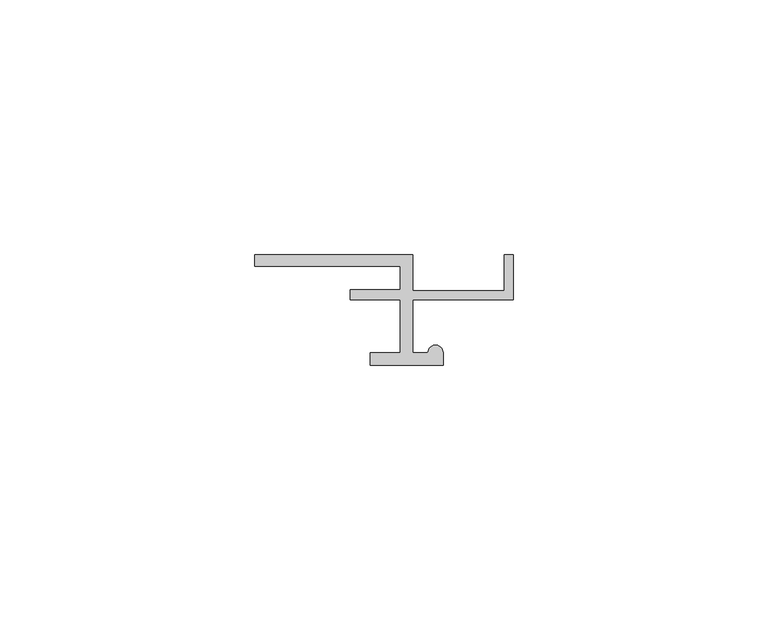
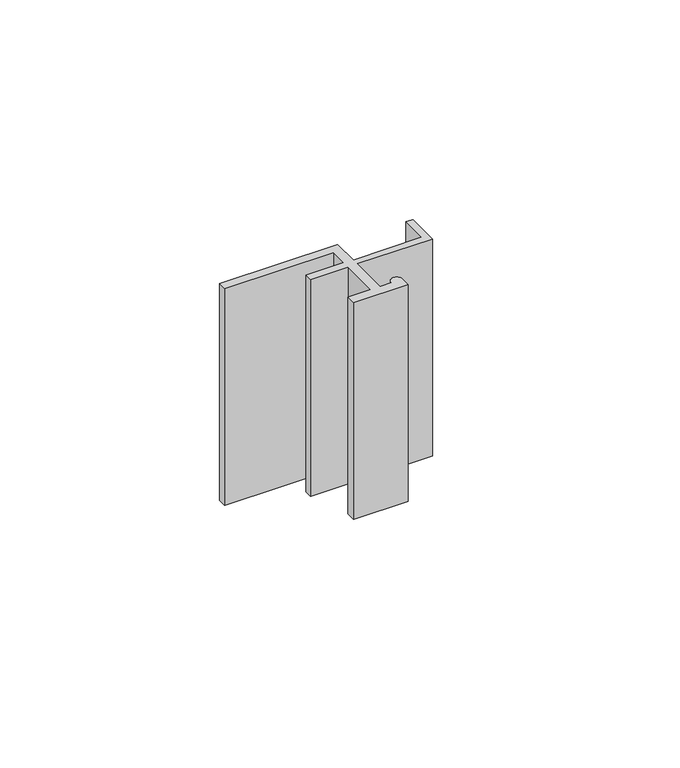
"""IFC4 building model written with IfcOpenShell, lengths in millimetres: proxy geometry, Generic Models 9:Generic Models 5:348123:Generic Models 5:348123 : Generic Models 9:Generic Models 5:348123:3 : Generic Models 9:Generic Models 5:348123:Generic Models 5:348123 : Generic Models 9:Generic Models 5:348123:301771."""

from ifc_helpers import new_model, si_unit, point, frame, frame_2d, origin, place, context, project, spatial, polyline, circle_curve, trimmed, segment, composite_curve, outline, extrude, source, transform, mapped, element, save


def generic_models_26c4c3e7(model_context):
    return source(origin(), model_context, "Body", "SweptSolid", [
        extrude(outline(composite_curve([segment(polyline([(593310.4802827, -568228.176062), (593310.4802827, -568238.5333435), (593313.439506, -568238.5333435)]), True, "CONTINUOUS"), segment(trimmed(circle_curve(frame_2d((593314.9191176, -568238.5333435)), 1.4796117), [point((593313.439506, -568238.5333435))], [point((593316.3987293, -568238.5333435))], False, "CARTESIAN"), True, "CONTINUOUS"), segment(polyline([(593316.3987293, -568238.5333435), (593316.3987293, -568240.9993629), (593302.0958166, -568240.9993629), (593302.0958166, -568238.5333435), (593308.0142632, -568238.5333435), (593308.0142632, -568228.176062), (593298.1501856, -568228.176062), (593298.1501856, -568226.2032464), (593308.0142632, -568226.2032464), (593308.0142632, -568221.5671299), (593279.408438, -568221.5671299), (593279.408438, -568219.2983921), (593310.4802827, -568219.2983921), (593310.4802827, -568226.400528), (593328.432904, -568226.400528), (593328.432904, -568219.2983921), (593330.208438, -568219.2983921), (593330.208438, -568228.176062), (593310.4802827, -568228.176062)]), True, "CONTINUOUS")], self_intersect=False)), frame((0.0, 0.0, 6059.090625), z_axis=(0.0, 0.0, 1.0), x_axis=(1.0, 0.0, 0.0)), (0.0, 0.0, 1.0), 60.325),
    ])


if __name__ == "__main__":
    model = new_model("IFC4")
    model_context = context("Model", 3, world=origin())
    ifc_project = project(units=[si_unit("LENGTHUNIT", "METRE", prefix="MILLI")], contexts=[model_context])
    site = spatial("IfcSite", under=ifc_project)
    building = spatial("IfcBuilding", under=site)
    placement = place(None, origin())
    generic_models_shape = generic_models_26c4c3e7(model_context)
    element("IfcBuildingElementProxy", 1, Name="Generic Models 9:Generic Models 5:348123:Generic Models 5:348123 : Generic Models 9:Generic Models 5:348123:3 : Generic Models 9:Generic Models 5:348123:Generic Models 5:348123 : Generic Models 9:Generic Models 5:348123:301771", ObjectType="Generic Models 9:Generic Models 5:348123:Generic Models 5:348123 : Generic Models 9:Generic Models 5:348123:3 : Generic Models 9:Generic Models 5:348123:Generic Models 5:348123 : Generic Models 9:Generic Models 5:348123:301771", at=placement, inside=building, context=model_context, shape_type="MappedRepresentation", body=[
        mapped(generic_models_shape, transform((0.0, 0.0, 0.0), x_axis=(1.0, 0.0, 0.0), y_axis=(0.0, 1.0, 0.0), z_axis=(0.0, 0.0, 1.0))),
    ])
    save(model, "model.ifc")

# Revit data of these elements
# Type "Generic Models 9:Generic Models 5:348123:Generic Models 5:348123 : Generic Models 9:Generic Models 5:348123:3 : Generic Models 9:Generic Models 5:348123:Generic Models 5:348123 : Generic Models 9:Generic Models 5:348123:301771"
#   NameOverride = "Generic Models 9:Generic Models 5:348123:Generic Models 5:348123 : Generic Models 9:Generic Models 5:348123:301771"
#   ObjectTypeOverride = "Generic Models 5:348123 : Generic Models 9:Generic Models 5:348123"
#   Reference = "Generic Models 5"
#   Tag = "301771"
# Element 1 (IfcBuildingElementProxy, "Generic Models 9:Generic Models 5:348123:Generic Models 5:348123 : Generic Models 9:Generic Models 5:348123:3 : Generic Models 9:Generic Models 5:348123:Generic Models 5:348123 : Generic Models 9:Generic Models 5:348123:301771")
#   Materials on its faces: "GA. STEEL CLIP AT EVERY SEAM IN POLYCARBONATE (WITH STEEL PLATE EXTENSION, IF NECS.)"
# Materials
#   "GA. STEEL CLIP AT EVERY SEAM IN POLYCARBONATE (WITH STEEL PLATE EXTENSION, IF NECS.)": class "Unassigned", colour RGB 120 120 120, transparency 0, Cost = 0
